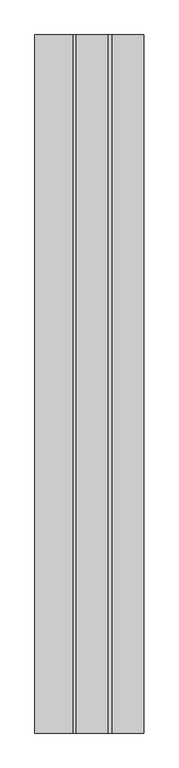
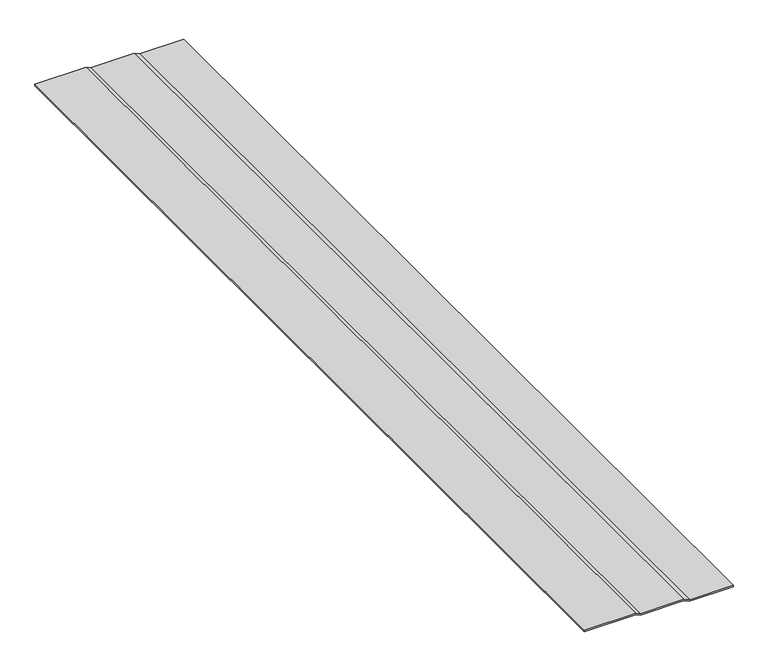
"""IFC4 building model written with IfcOpenShell, lengths in millimetres: proxy geometry, BITUMEN CAP SHEET001 3829 : BITUMEN CAP SHEET001 3829."""

import ifcopenshell
import ifcopenshell.guid

model = None  # the IFC model being written
_history = None  # IfcOwnerHistory: only IFC2X3 demands one
_inside = {}  # id of a spatial element -> (the spatial element, [elements in it])
_under = {}  # id of a project, library or spatial element -> (it, [spatial elements below it])
_declared = {}  # id of a project -> (the project, [libraries it declares])
_typed = {}  # id of a type object -> (the type object, [elements of that type])
_made_of = {}  # id of a material, layer set ... -> (it, [elements and type objects made of it])


def new_model(schema):
    """Start an empty IFC model of exactly this schema.

    Asked for "IFC4X3", IfcOpenShell would pick the latest addendum, in which some entities
    have other attributes; the version numbers below select the first issue.
    IFC2X3 requires an IfcOwnerHistory on every rooted entity: one is made here for all.
    """
    global model, _history
    if schema == "IFC4X3":
        model = ifcopenshell.file(schema_version=(4, 3, 0, 0))
    else:
        model = ifcopenshell.file(schema=schema)
    _inside.clear()
    _under.clear()
    _declared.clear()
    _typed.clear()
    _made_of.clear()
    _history = None
    if model.schema == "IFC2X3":
        org = make("IfcOrganization", Name="unknown")
        user = make(
            "IfcPersonAndOrganization",
            ThePerson=make("IfcPerson", FamilyName="unknown"),
            TheOrganization=org,
        )
        app = make(
            "IfcApplication",
            ApplicationDeveloper=org,
            Version="unknown",
            ApplicationFullName="unknown",
            ApplicationIdentifier="unknown",
        )
        _history = make(
            "IfcOwnerHistory",
            OwningUser=user,
            OwningApplication=app,
            ChangeAction="ADDED",
            CreationDate=0,
        )
    return model


def make(cls, **values):
    """One entity of the class cls with the attributes given. An attribute that is None is left unset."""
    return model.create_entity(
        cls, **{name: value for name, value in values.items() if value is not None}
    )


def rooted(cls, **values):
    """An entity with a GlobalId (a new one), such as an element, a storey or a relation."""
    return make(cls, GlobalId=ifcopenshell.guid.new(), OwnerHistory=_history, **values)


def si_unit(unit_type, name, prefix=None):
    """IfcSIUnit, for example si_unit("LENGTHUNIT", "METRE", prefix="MILLI")."""
    return make("IfcSIUnit", UnitType=unit_type, Prefix=prefix, Name=name)


def assignment(units):
    """IfcUnitAssignment: the units of a project."""
    return None if units is None else make("IfcUnitAssignment", Units=units)


def point(xyz):
    """IfcCartesianPoint."""
    return None if xyz is None else make("IfcCartesianPoint", Coordinates=xyz)


def direction(xyz):
    """IfcDirection."""
    return None if xyz is None else make("IfcDirection", DirectionRatios=xyz)


def frame(location, z_axis=None, x_axis=None):
    """IfcAxis2Placement3D, a coordinate frame: its origin and axes. An axis left out is left unset."""
    return make(
        "IfcAxis2Placement3D",
        Location=point(location),
        Axis=direction(z_axis),
        RefDirection=direction(x_axis),
    )


def origin():
    """The frame at (0, 0, 0) with its axes left unset."""
    return frame((0.0, 0.0, 0.0))


def place(relative_to, where):
    """IfcLocalPlacement: puts the frame where relative to a parent placement (None: the world)."""
    return make(
        "IfcLocalPlacement", PlacementRelTo=relative_to, RelativePlacement=where
    )


def context(
    kind, dimensions, precision=None, world=None, true_north=None, identifier=None
):
    """IfcGeometricRepresentationContext, for example the 3D "Model" context."""
    return make(
        "IfcGeometricRepresentationContext",
        ContextIdentifier=identifier,
        ContextType=kind,
        CoordinateSpaceDimension=dimensions,
        Precision=precision,
        WorldCoordinateSystem=world,
        TrueNorth=true_north,
    )


def project(units=None, contexts=None):
    """IfcProject with its units and contexts."""
    return rooted(
        "IfcProject",
        Name="project",
        RepresentationContexts=contexts,
        UnitsInContext=assignment(units),
    )


def spatial(cls, under=None, at=None, **own):
    """A site, building, storey or space (cls), placed at a placement, below another one or the project."""
    s = rooted(cls, ObjectPlacement=at, **own)
    if under is not None:
        _under.setdefault(under.id(), (under, []))[1].append(s)
    return s


def polyline(points):
    """IfcPolyline through the points."""
    return make("IfcPolyline", Points=[point(p) for p in points])


def outline(outer, holes=None, kind="AREA"):
    """IfcArbitraryClosedProfileDef: a profile drawn as a closed curve; with holes, ...WithVoids."""
    if holes is None:
        return make("IfcArbitraryClosedProfileDef", ProfileType=kind, OuterCurve=outer)
    return make(
        "IfcArbitraryProfileDefWithVoids",
        ProfileType=kind,
        OuterCurve=outer,
        InnerCurves=holes,
    )


def extrude(swept, where, along, depth):
    """IfcExtrudedAreaSolid: the profile swept, set in the frame where, extruded along a direction by depth."""
    return make(
        "IfcExtrudedAreaSolid",
        SweptArea=swept,
        Position=where,
        ExtrudedDirection=direction(along),
        Depth=depth,
    )


def shape(context_of_items, identifier, shape_type, items):
    """IfcShapeRepresentation: the items that make up one representation, for example the "Body"."""
    return make(
        "IfcShapeRepresentation",
        ContextOfItems=context_of_items,
        RepresentationIdentifier=identifier,
        RepresentationType=shape_type,
        Items=items,
    )


def source(mapping_origin, context_of_items, identifier, shape_type, items):
    """IfcRepresentationMap: a shape defined once, which mapped items show again and again."""
    return make(
        "IfcRepresentationMap",
        MappingOrigin=mapping_origin,
        MappedRepresentation=shape(context_of_items, identifier, shape_type, items),
    )


def transform(
    local_origin,
    x_axis=None,
    y_axis=None,
    z_axis=None,
    scale=None,
    scale2=None,
    scale3=None,
    uniform=True,
):
    """IfcCartesianTransformationOperator3D, or its non-uniform kind. x_axis, y_axis, z_axis: its Axis1, 2, 3."""
    if uniform:
        return make(
            "IfcCartesianTransformationOperator3D",
            Axis1=direction(x_axis),
            Axis2=direction(y_axis),
            LocalOrigin=point(local_origin),
            Scale=scale,
            Axis3=direction(z_axis),
        )
    return make(
        "IfcCartesianTransformationOperator3DnonUniform",
        Axis1=direction(x_axis),
        Axis2=direction(y_axis),
        LocalOrigin=point(local_origin),
        Scale=scale,
        Axis3=direction(z_axis),
        Scale2=scale2,
        Scale3=scale3,
    )


def mapped(mapping_source, mapping_target):
    """IfcMappedItem: shows the shape of a source again, moved by a transform."""
    return make(
        "IfcMappedItem", MappingSource=mapping_source, MappingTarget=mapping_target
    )


def made_of(thing, what):
    """Note that an element or type object is made of a material, layer set ...; save() writes the relation."""
    if what is not None:
        _made_of.setdefault(what.id(), (what, []))[1].append(thing)
    return thing


def element(
    cls,
    number,
    at=None,
    inside=None,
    cuts=None,
    type_object=None,
    material=None,
    context=None,
    identifier="Body",
    shape_type=None,
    held_by="IfcProductDefinitionShape",
    body=None,
    shapes=None,
    **own,
):
    """One element of the class cls, such as IfcWall. Its Tag is "e" and its number.

    at: its placement. inside: the storey or other place that contains it. cuts: it is an
    opening in that element (IfcRelVoidsElement). A single representation is given by context,
    identifier, shape_type and body (its items); several are given by shapes. held_by: the class
    of the entity that holds the representations. save() writes the other relations.
    """
    e = rooted(cls, Tag="e%d" % number, ObjectPlacement=at, **own)
    if body is not None:
        shapes = [shape(context, identifier, shape_type, body)]
    if shapes is not None:
        e.Representation = make(held_by, Representations=shapes)
    if inside is not None:
        _inside.setdefault(inside.id(), (inside, []))[1].append(e)
    if cuts is not None:
        rooted(
            "IfcRelVoidsElement", RelatingBuildingElement=cuts, RelatedOpeningElement=e
        )
    if type_object is not None:
        _typed.setdefault(type_object.id(), (type_object, []))[1].append(e)
    return made_of(e, material)


def aggregate(whole, parts):
    """IfcRelAggregates: a whole, such as a stair, and the parts it consists of."""
    return rooted("IfcRelAggregates", RelatingObject=whole, RelatedObjects=parts)


def save(model, path):
    """Write the relations noted so far, then the file.

    IfcRelAggregates (storeys below a building ...), IfcRelContainedInSpatialStructure (elements
    in a storey), IfcRelDefinesByType, IfcRelAssociatesMaterial and IfcRelDeclares: one each for
    every whole, place, type object, material and project.
    """
    for whole, parts in _under.values():
        aggregate(whole, parts)
    for where, things in _inside.values():
        rooted(
            "IfcRelContainedInSpatialStructure",
            RelatedElements=things,
            RelatingStructure=where,
        )
    for kind, things in _typed.values():
        rooted("IfcRelDefinesByType", RelatedObjects=things, RelatingType=kind)
    for what, things in _made_of.values():
        rooted("IfcRelAssociatesMaterial", RelatedObjects=things, RelatingMaterial=what)
    for by, libraries in _declared.values():
        rooted("IfcRelDeclares", RelatingContext=by, RelatedDefinitions=libraries)
    model.write(path)


def generic_models_3f8c56e2(model_context):
    return source(origin(), model_context, "Body", "SweptSolid", [
        extrude(outline(polyline([(40259.2002678, -4699.8063764), (40262.3752678, -4699.8063764), (40262.3752678, -4791.325638), (40267.6612773, -4803.7904566), (40267.6612773, -4894.4742123), (40271.9940719, -4904.1911138), (40271.9940719, -5012.0776104), (40268.8188423, -5012.0776104), (40268.8188423, -4904.8663993), (40264.4862773, -4895.1500128), (40264.4862773, -4804.4358566), (40259.2002678, -4791.971038), (40259.2002678, -4699.8063764)])), frame((0.0, -1052.8906574, 0.0), z_axis=(0.0, 1.0, 0.0), x_axis=(0.0, 0.0, 1.0)), (0.0, 0.0, 1.0), 2000.25),
    ])


if __name__ == "__main__":
    model = new_model("IFC4")
    model_context = context("Model", 3, world=origin())
    ifc_project = project(units=[si_unit("LENGTHUNIT", "METRE", prefix="MILLI")], contexts=[model_context])
    site = spatial("IfcSite", under=ifc_project)
    building = spatial("IfcBuilding", under=site)
    placement = place(None, origin())
    generic_models_shape = generic_models_3f8c56e2(model_context)
    element("IfcBuildingElementProxy", 1, Name="BITUMEN CAP SHEET001 3829 : BITUMEN CAP SHEET001 3829", ObjectType="BITUMEN CAP SHEET001 3829 : BITUMEN CAP SHEET001 3829", at=placement, inside=building, context=model_context, shape_type="MappedRepresentation", body=[
        mapped(generic_models_shape, transform((0.0, 0.0, 0.0), x_axis=(1.0, 0.0, 0.0), y_axis=(0.0, 1.0, 0.0), z_axis=(0.0, 0.0, 1.0))),
    ])
    save(model, "model.ifc")

# Revit data of these elements
# Type "BITUMEN CAP SHEET001 3829 : BITUMEN CAP SHEET001 3829"
#   NameOverride = "BITUMEN CAP SHEET001"
# Element 1 (IfcBuildingElementProxy, "BITUMEN CAP SHEET001 3829 : BITUMEN CAP SHEET001 3829")
#   Materials on its faces: "MODIFIED BITUMEN GRANULE SURFACED CAP SHEET"
# Materials
#   "MODIFIED BITUMEN GRANULE SURFACED CAP SHEET": class "Unassigned", colour RGB 85 85 127, transparency 0
